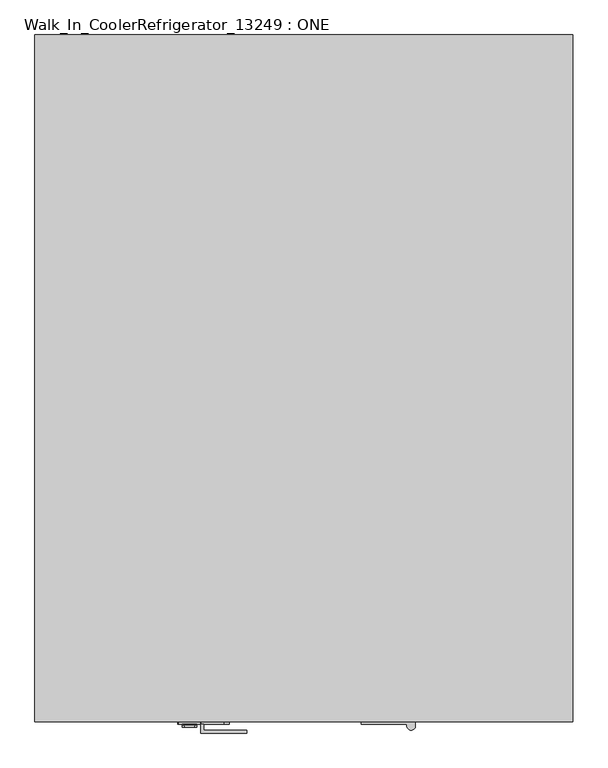
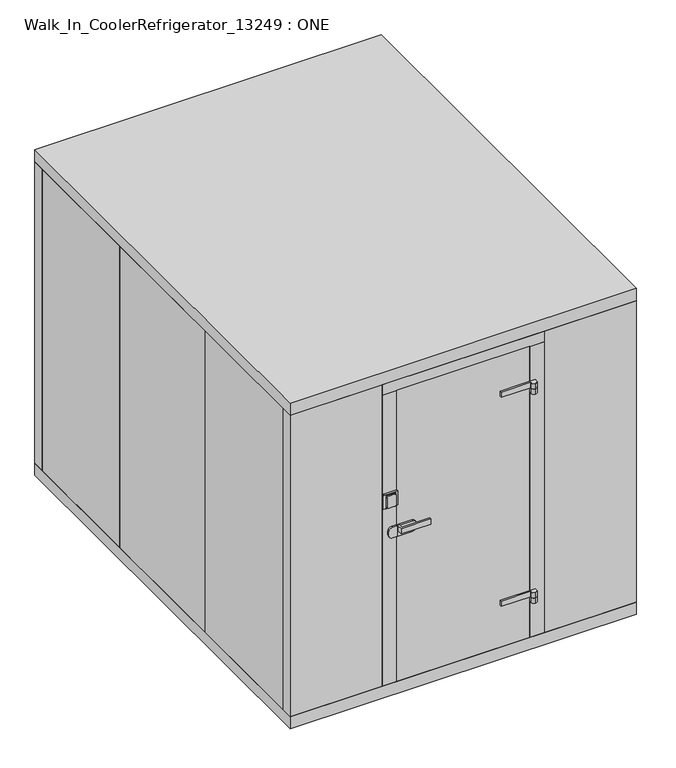
"""IFC4 building model written with IfcOpenShell, lengths in millimetres: proxy geometry, Walk_In_CoolerRefrigerator_13249 : ONE."""

from ifc_helpers import new_model, si_unit, point, frame, frame_2d, origin, origin_with_axes, place, context, project, spatial, polyline, circle_curve, trimmed, segment, composite_curve, outline, extrude, source, transform, mapped, element, save
from ifc_brep_helpers import plane_surface, cylinder_surface, spline_surface, advanced_brep


def walk_in_coolerrefrigerator_13249_one_21fe9a68(model_context):
    return source(origin(), model_context, "Body", "SolidModel", [
        advanced_brep(
        [(-488.8645847, -1549.4, 1390.65), (-527.1354153, -1549.4, 1390.65), (-539.8354153, -1549.4, 1377.95), (-539.8354153, -1549.4, 1314.45), (-527.1354153, -1549.4, 1301.75), (-488.8645847, -1549.4, 1301.75), (-476.1645847, -1549.4, 1314.45), (-476.1645847, -1549.4, 1377.95), (-482.5145847, -1539.875, 1390.65), (-476.1645847, -1539.875, 1384.3), (-476.1645847, -1539.875, 1308.1), (-482.5145847, -1539.875, 1301.75), (-533.4854153, -1539.875, 1301.75), (-539.8354153, -1539.875, 1308.1), (-539.8354153, -1539.875, 1384.3), (-533.4854153, -1539.875, 1390.65)],
        [
            (0, 1),
            (1, 2, circle_curve(frame((-527.1354153, -1549.4, 1377.95), z_axis=(0.0, -1.0, 0.0), x_axis=(-1.0, 0.0, 0.0)), 12.7)),
            (2, 3),
            (3, 4, circle_curve(frame((-527.1354153, -1549.4, 1314.45), z_axis=(0.0, -1.0, 0.0), x_axis=(-1.0, 0.0, 0.0)), 12.7)),
            (4, 5),
            (5, 6, circle_curve(frame((-488.8645847, -1549.4, 1314.45), z_axis=(0.0, -1.0, 0.0), x_axis=(-1.0, 0.0, 0.0)), 12.7)),
            (6, 7),
            (7, 0, circle_curve(frame((-488.8645847, -1549.4, 1377.95), z_axis=(0.0, -1.0, 0.0), x_axis=(-1.0, 0.0, 0.0)), 12.7)),
            (8, 9, circle_curve(frame((-482.5145847, -1539.875, 1384.3), z_axis=(0.0, 1.0, 0.0), x_axis=(-1.0, 0.0, 0.0)), 6.35)),
            (9, 10),
            (10, 11, circle_curve(frame((-482.5145847, -1539.875, 1308.1), z_axis=(0.0, 1.0, 0.0), x_axis=(-1.0, 0.0, 0.0)), 6.35)),
            (11, 12),
            (12, 13, circle_curve(frame((-533.4854153, -1539.875, 1308.1), z_axis=(0.0, 1.0, 0.0), x_axis=(-1.0, 0.0, 0.0)), 6.35)),
            (13, 14),
            (14, 15, circle_curve(frame((-533.4854153, -1539.875, 1384.3), z_axis=(0.0, 1.0, 0.0), x_axis=(-1.0, 0.0, 0.0)), 6.35)),
            (15, 8),
            (15, 1),
            (0, 8),
            (14, 2),
            (13, 3),
            (12, 4),
            (11, 5),
            (10, 6),
            (9, 7),
        ],
        [
            plane_surface(frame((-508.0, -1549.4, 1346.2), z_axis=(0.0, -1.0, 0.0), x_axis=(-1.0, 0.0, 0.0))),
            plane_surface(frame((-508.0, -1539.875, 1346.2), z_axis=(0.0, 1.0, 0.0), x_axis=(-1.0, 0.0, 0.0))),
            plane_surface(frame((-508.0, -1539.875, 1390.65), z_axis=(0.0, 0.0, 1.0), x_axis=(-1.0, 0.0, 0.0))),
            spline_surface(2, 1, [[(-533.4854153, -1539.875, 1390.65), (-527.1354153, -1549.4, 1390.65)], [(-539.8354153000001, -1539.875, 1390.65), (-539.8354153, -1549.4, 1390.65)], [(-539.8354153, -1539.875, 1384.3), (-539.8354153, -1549.4, 1377.95)]], [3, 3], [2, 2], [0.0, 1.0], [0.0, 1.0], weights=[[1.0, 1.0], [0.7071067811865476, 0.7071067811865476], [1.0, 1.0]]),
            plane_surface(frame((-539.8354153, -1539.875, 1346.2), z_axis=(-1.0, 0.0, 0.0), x_axis=(0.0, 0.0, -1.0))),
            spline_surface(2, 1, [[(-539.8354153, -1539.875, 1308.1), (-539.8354153, -1549.4, 1314.45)], [(-539.8354153, -1539.875, 1301.75), (-539.8354153, -1549.4, 1301.75)], [(-533.4854153, -1539.875, 1301.75), (-527.1354153, -1549.4, 1301.75)]], [3, 3], [2, 2], [0.0, 1.0], [0.0, 1.0], weights=[[1.0, 1.0], [0.7071067811865476, 0.7071067811865476], [1.0, 1.0]]),
            plane_surface(frame((-508.0, -1539.875, 1301.75), z_axis=(0.0, 0.0, -1.0), x_axis=(1.0, 0.0, 0.0))),
            spline_surface(2, 1, [[(-482.5145847, -1539.875, 1301.75), (-488.8645847, -1549.4, 1301.75)], [(-476.1645847000001, -1539.875, 1301.75), (-476.1645847, -1549.4, 1301.75)], [(-476.1645847, -1539.875, 1308.1), (-476.1645847, -1549.4, 1314.45)]], [3, 3], [2, 2], [0.0, 1.0], [0.0, 1.0], weights=[[1.0, 1.0], [0.7071067811865476, 0.7071067811865476], [1.0, 1.0]]),
            plane_surface(frame((-476.1645847, -1539.875, 1346.2), z_axis=(1.0, 0.0, 0.0), x_axis=(0.0, 0.0, 1.0))),
            spline_surface(2, 1, [[(-476.1645847, -1539.875, 1384.3), (-476.1645847, -1549.4, 1377.95)], [(-476.1645847, -1539.875, 1390.65), (-476.1645847, -1549.4, 1390.65)], [(-482.5145847, -1539.875, 1390.65), (-488.8645847, -1549.4, 1390.65)]], [3, 3], [2, 2], [0.0, 1.0], [0.0, 1.0], weights=[[1.0, 1.0], [0.7071067811865476, 0.7071067811865476], [1.0, 1.0]]),
        ],
        [
            (0, [[1, 2, 3, 4, 5, 6, 7, 8]]),
            (1, [[9, 10, 11, 12, 13, 14, 15, 16]]),
            (2, [[-16, 17, -1, 18]]),
            (3, [[-15, 19, -2, -17]]),
            (4, [[-14, 20, -3, -19]]),
            (5, [[-13, 21, -4, -20]]),
            (6, [[-12, 22, -5, -21]]),
            (7, [[-11, 23, -6, -22]]),
            (8, [[-10, 24, -7, -23]]),
            (9, [[-9, -18, -8, -24]]),
        ],
    ),
        advanced_brep(
        [(-555.625, -1536.7, 1397.0), (-558.8, -1536.7, 1393.825), (-558.8, -1536.7, 1298.575), (-555.625, -1536.7, 1295.4), (-539.8354153, -1536.7, 1295.4), (-539.8354153, -1536.7, 1397.0), (-460.375, -1536.7, 1295.4), (-457.2, -1536.7, 1298.575), (-457.2, -1536.7, 1393.825), (-460.375, -1536.7, 1397.0), (-476.1645847, -1536.7, 1397.0), (-476.1645847, -1536.7, 1295.4), (-460.375, -1524.0, 1397.0), (-457.2, -1524.0, 1393.825), (-457.2, -1524.0, 1298.575), (-460.375, -1524.0, 1295.4), (-555.625, -1524.0, 1295.4), (-558.8, -1524.0, 1298.575), (-558.8, -1524.0, 1393.825), (-555.625, -1524.0, 1397.0), (-476.1645847, -1539.875, 1390.65), (-539.8354153, -1539.875, 1390.65), (-539.8354153, -1539.875, 1301.75), (-476.1645847, -1539.875, 1301.75)],
        [
            (0, 1, circle_curve(frame((-555.625, -1536.7, 1393.825), z_axis=(0.0, -1.0, 0.0), x_axis=(-1.0, 0.0, 0.0)), 3.175)),
            (1, 2),
            (2, 3, circle_curve(frame((-555.625, -1536.7, 1298.575), z_axis=(0.0, -1.0, 0.0), x_axis=(-1.0, 0.0, 0.0)), 3.175)),
            (3, 4),
            (4, 5),
            (5, 0),
            (6, 7, circle_curve(frame((-460.375, -1536.7, 1298.575), z_axis=(0.0, -1.0, 0.0), x_axis=(-1.0, 0.0, 0.0)), 3.175)),
            (7, 8),
            (8, 9, circle_curve(frame((-460.375, -1536.7, 1393.825), z_axis=(0.0, -1.0, 0.0), x_axis=(-1.0, 0.0, 0.0)), 3.175)),
            (9, 10),
            (10, 11),
            (11, 6),
            (12, 13, circle_curve(frame((-460.375, -1524.0, 1393.825), z_axis=(0.0, 1.0, 0.0), x_axis=(-1.0, 0.0, 0.0)), 3.175)),
            (13, 14),
            (14, 15, circle_curve(frame((-460.375, -1524.0, 1298.575), z_axis=(0.0, 1.0, 0.0), x_axis=(-1.0, 0.0, 0.0)), 3.175)),
            (15, 16),
            (16, 17, circle_curve(frame((-555.625, -1524.0, 1298.575), z_axis=(0.0, 1.0, 0.0), x_axis=(-1.0, 0.0, 0.0)), 3.175)),
            (17, 18),
            (18, 19, circle_curve(frame((-555.625, -1524.0, 1393.825), z_axis=(0.0, 1.0, 0.0), x_axis=(-1.0, 0.0, 0.0)), 3.175)),
            (19, 12),
            (19, 0),
            (5, 10),
            (9, 12),
            (18, 1),
            (17, 2),
            (16, 3),
            (15, 6),
            (11, 4),
            (14, 7),
            (13, 8),
            (20, 21),
            (21, 22),
            (22, 23),
            (23, 20),
            (20, 10),
            (5, 21),
            (4, 22),
            (11, 23),
        ],
        [
            plane_surface(frame((-555.625, -1536.7, 1397.0), z_axis=(0.0, -1.0, 0.0), x_axis=(-1.0, 0.0, 0.0))),
            plane_surface(frame((-555.625, -1524.0, 1397.0), z_axis=(0.0, 1.0, 0.0), x_axis=(1.0, 0.0, 0.0))),
            plane_surface(frame((-460.375, -1536.7, 1397.0), z_axis=(0.0, 0.0, 1.0), x_axis=(0.0, 1.0, 0.0))),
            cylinder_surface(frame((-555.625, -1524.0, 1393.825), z_axis=(0.0, -1.0, 0.0), x_axis=(-1.0, 0.0, 0.0)), 3.175),
            plane_surface(frame((-558.8, -1536.7, 1393.825), z_axis=(-1.0, 0.0, 0.0), x_axis=(0.0, 1.0, 0.0))),
            cylinder_surface(frame((-555.625, -1524.0, 1298.575), z_axis=(0.0, -1.0, 0.0), x_axis=(-1.0, 0.0, 0.0)), 3.175),
            plane_surface(frame((-555.625, -1536.7, 1295.4), z_axis=(0.0, 0.0, -1.0), x_axis=(0.0, 1.0, 0.0))),
            cylinder_surface(frame((-460.375, -1524.0, 1298.575), z_axis=(0.0, -1.0, 0.0), x_axis=(-1.0, 0.0, 0.0)), 3.175),
            plane_surface(frame((-457.2, -1536.7, 1298.575), z_axis=(1.0, 0.0, 0.0), x_axis=(0.0, 1.0, 0.0))),
            cylinder_surface(frame((-460.375, -1524.0, 1393.825), z_axis=(0.0, -1.0, 0.0), x_axis=(-1.0, 0.0, 0.0)), 3.175),
            plane_surface(frame((-508.0, -1539.875, 1346.2), z_axis=(0.0, -1.0, 0.0), x_axis=(-1.0, 0.0, 0.0))),
            plane_surface(frame((-508.0, -1536.7, 1397.0), z_axis=(0.0, -0.8944271909999134, 0.447213595499963), x_axis=(-1.0, 0.0, 0.0))),
            plane_surface(frame((-539.8354153, -1536.7, 1346.2), z_axis=(-1.0, 0.0, 0.0), x_axis=(0.0, 0.0, -1.0))),
            plane_surface(frame((-508.0, -1536.7, 1295.4), z_axis=(0.0, -0.8944271909999666, -0.4472135954998567), x_axis=(1.0, 0.0, 0.0))),
            plane_surface(frame((-476.1645847, -1536.7, 1346.2), z_axis=(1.0, 0.0, 0.0), x_axis=(0.0, 0.0, 1.0))),
        ],
        [
            (0, [[1, 2, 3, 4, 5, 6]]),
            (0, [[7, 8, 9, 10, 11, 12]]),
            (1, [[13, 14, 15, 16, 17, 18, 19, 20]]),
            (2, [[-20, 21, -6, 22, -10, 23]]),
            (3, [[-1, -21, -19, 24]]),
            (4, [[-2, -24, -18, 25]]),
            (5, [[-3, -25, -17, 26]]),
            (6, [[-16, 27, -12, 28, -4, -26]]),
            (7, [[-7, -27, -15, 29]]),
            (8, [[-8, -29, -14, 30]]),
            (9, [[-9, -30, -13, -23]]),
            (10, [[31, 32, 33, 34]]),
            (11, [[-31, 35, -22, 36]]),
            (12, [[-32, -36, -5, 37]]),
            (13, [[-33, -37, -28, 38]]),
            (14, [[-34, -38, -11, -35]]),
        ],
    ),
        extrude(outline(polyline([(-457.2, -1574.8), (-457.2, -1536.7), (-444.5, -1536.7), (-444.5, -1562.1), (-254.0, -1562.1), (-254.0, -1574.8), (-457.2, -1574.8)])), frame((0.0, 0.0, 1104.9), z_axis=(0.0, 0.0, 1.0), x_axis=(1.0, 0.0, 0.0)), (0.0, 0.0, 1.0), 38.1),
        extrude(outline(composite_curve([segment(polyline([(1066.8, -457.2), (1066.8, -355.6)]), True, "CONTINUOUS"), segment(trimmed(circle_curve(frame_2d((1092.2, -355.6)), 25.4), [point((1066.8, -355.6))], [point((1092.2, -330.2))], False, "CARTESIAN"), True, "CONTINUOUS"), segment(polyline([(1092.2, -330.2), (1117.6, -330.2)]), True, "CONTINUOUS"), segment(trimmed(circle_curve(frame_2d((1117.6, -355.6)), 25.4), [point((1117.6, -330.2))], [point((1143.0, -355.6))], False, "CARTESIAN"), True, "CONTINUOUS"), segment(polyline([(1143.0, -355.6), (1143.0, -457.2), (1066.8, -457.2)]), True, "CONTINUOUS")], self_intersect=False)), frame((0.0, -1536.7, 0.0), z_axis=(0.0, 1.0, 0.0), x_axis=(0.0, 0.0, 1.0)), (0.0, 0.0, 1.0), 12.7),
        extrude(outline(composite_curve([segment(polyline([(1066.8, -457.2), (1143.0, -457.2), (1143.0, -495.3)]), True, "CONTINUOUS"), segment(trimmed(circle_curve(frame_2d((1117.6, -495.3)), 25.4), [point((1143.0, -495.3))], [point((1117.6, -520.7))], False, "CARTESIAN"), True, "CONTINUOUS"), segment(polyline([(1117.6, -520.7), (1092.2, -520.7)]), True, "CONTINUOUS"), segment(trimmed(circle_curve(frame_2d((1092.2, -495.3)), 25.4), [point((1092.2, -520.7))], [point((1066.8, -495.3))], False, "CARTESIAN"), True, "CONTINUOUS"), segment(polyline([(1066.8, -495.3), (1066.8, -457.2)]), True, "CONTINUOUS")], self_intersect=False)), frame((0.0, -1536.7, 0.0), z_axis=(0.0, 1.0, 0.0), x_axis=(0.0, 0.0, 1.0)), (0.0, 0.0, 1.0), 12.7),
        extrude(outline(composite_curve([segment(polyline([(254.0, -1536.7), (254.0, -1524.0), (495.3, -1524.0), (495.3, -1543.05)]), True, "CONTINUOUS"), segment(trimmed(circle_curve(frame_2d((476.25, -1543.05)), 19.05), [point((495.3, -1543.05))], [point((476.25, -1562.1))], False, "CARTESIAN"), True, "CONTINUOUS"), segment(trimmed(circle_curve(frame_2d((476.25, -1543.05)), 19.05), [point((476.25, -1562.1))], [point((457.2, -1543.05))], False, "CARTESIAN"), True, "CONTINUOUS"), segment(polyline([(457.2, -1543.05), (457.2, -1536.7), (254.0, -1536.7)]), True, "CONTINUOUS")], self_intersect=False)), frame((0.0, 0.0, 304.8), z_axis=(0.0, 0.0, 1.0), x_axis=(1.0, 0.0, 0.0)), (0.0, 0.0, 1.0), 38.1),
        extrude(outline(composite_curve([segment(polyline([(457.2, -1543.05), (457.2, -1524.0), (495.3, -1524.0), (495.3, -1543.05)]), True, "CONTINUOUS"), segment(trimmed(circle_curve(frame_2d((476.25, -1543.05)), 19.05), [point((495.3, -1543.05))], [point((476.25, -1562.1))], False, "CARTESIAN"), True, "CONTINUOUS"), segment(trimmed(circle_curve(frame_2d((476.25, -1543.05)), 19.05), [point((476.25, -1562.1))], [point((457.2, -1543.05))], False, "CARTESIAN"), True, "CONTINUOUS")], self_intersect=False)), frame((0.0, 0.0, 266.7), z_axis=(0.0, 0.0, 1.0), x_axis=(1.0, 0.0, 0.0)), (0.0, 0.0, 1.0), 38.1),
        extrude(outline(composite_curve([segment(polyline([(495.3, -1524.0), (495.3, -1543.05)]), True, "CONTINUOUS"), segment(trimmed(circle_curve(frame_2d((476.25, -1543.05)), 19.05), [point((495.3, -1543.05))], [point((476.25, -1562.1))], False, "CARTESIAN"), True, "CONTINUOUS"), segment(trimmed(circle_curve(frame_2d((476.25, -1543.05)), 19.05), [point((476.25, -1562.1))], [point((457.2, -1543.05))], False, "CARTESIAN"), True, "CONTINUOUS"), segment(polyline([(457.2, -1543.05), (457.2, -1536.7), (254.0, -1536.7), (254.0, -1524.0), (495.3, -1524.0)]), True, "CONTINUOUS")], self_intersect=False)), frame((0.0, 0.0, 1828.8), z_axis=(0.0, 0.0, 1.0), x_axis=(1.0, 0.0, 0.0)), (0.0, 0.0, 1.0), 38.1),
        extrude(outline(composite_curve([segment(polyline([(457.2, -1543.05), (457.2, -1524.0), (495.3, -1524.0), (495.3, -1543.05)]), True, "CONTINUOUS"), segment(trimmed(circle_curve(frame_2d((476.25, -1543.05)), 19.05), [point((495.3, -1543.05))], [point((476.25, -1562.1))], False, "CARTESIAN"), True, "CONTINUOUS"), segment(trimmed(circle_curve(frame_2d((476.25, -1543.05)), 19.05), [point((476.25, -1562.1))], [point((457.2, -1543.05))], False, "CARTESIAN"), True, "CONTINUOUS")], self_intersect=False)), frame((0.0, 0.0, 1790.7), z_axis=(0.0, 0.0, 1.0), x_axis=(1.0, 0.0, 0.0)), (0.0, 0.0, 1.0), 38.1),
        extrude(outline(polyline([(457.2, -1435.1), (457.2, -1524.0), (-457.2, -1524.0), (-457.2, -1435.1), (457.2, -1435.1)])), origin_with_axes(), (0.0, 0.0, 1.0), 2120.9),
        extrude(outline(polyline([(558.8, -1435.1), (558.8, -1524.0), (-558.8, -1524.0), (-558.8, -1435.1), (558.8, -1435.1)])), frame((0.0, 0.0, 2120.9), z_axis=(0.0, 0.0, 1.0), x_axis=(1.0, 0.0, 0.0)), (0.0, 0.0, 1.0), 76.2),
        extrude(outline(polyline([(-558.8, -1435.1), (-457.2, -1435.1), (-457.2, -1524.0), (-558.8, -1524.0), (-558.8, -1435.1)])), origin_with_axes(), (0.0, 0.0, 1.0), 2120.9),
        extrude(outline(polyline([(558.8, -1435.1), (558.8, -1524.0), (457.2, -1524.0), (457.2, -1435.1), (558.8, -1435.1)])), origin_with_axes(), (0.0, 0.0, 1.0), 2120.9),
        extrude(outline(polyline([(1193.8, -1524.0), (-1193.8, -1524.0), (-1193.8, 1524.0), (1193.8, 1524.0), (1193.8, -1524.0)])), frame((0.0, 0.0, 2197.1), z_axis=(0.0, 0.0, 1.0), x_axis=(1.0, 0.0, 0.0)), (0.0, 0.0, 1.0), 88.9),
        extrude(outline(polyline([(-1193.8, -508.0), (-1104.9, -508.0), (-1104.9, -1435.1), (-1193.8, -1435.1), (-1193.8, -508.0)])), origin_with_axes(), (0.0, 0.0, 1.0), 2197.1),
        extrude(outline(polyline([(1104.9, -508.0), (1193.8, -508.0), (1193.8, -1435.1), (1104.9, -1435.1), (1104.9, -508.0)])), origin_with_axes(), (0.0, 0.0, 1.0), 2197.1),
        extrude(outline(polyline([(1104.9, 508.0), (1193.8, 508.0), (1193.8, -508.0), (1104.9, -508.0), (1104.9, 508.0)])), origin_with_axes(), (0.0, 0.0, 1.0), 2197.1),
        extrude(outline(polyline([(-1193.8, 508.0), (-1104.9, 508.0), (-1104.9, -508.0), (-1193.8, -508.0), (-1193.8, 508.0)])), origin_with_axes(), (0.0, 0.0, 1.0), 2197.1),
        extrude(outline(polyline([(-1193.8, 1435.1), (-1104.9, 1435.1), (-1104.9, 508.0), (-1193.8, 508.0), (-1193.8, 1435.1)])), origin_with_axes(), (0.0, 0.0, 1.0), 2197.1),
        extrude(outline(polyline([(1104.9, 1435.1), (1193.8, 1435.1), (1193.8, 508.0), (1104.9, 508.0), (1104.9, 1435.1)])), origin_with_axes(), (0.0, 0.0, 1.0), 2197.1),
        extrude(outline(polyline([(-457.2, 1435.1), (-457.2, 1524.0), (457.2, 1524.0), (457.2, 1435.1), (-457.2, 1435.1)])), origin_with_axes(), (0.0, 0.0, 1.0), 2197.1),
        extrude(outline(polyline([(457.2, 1435.1), (457.2, 1524.0), (1193.8, 1524.0), (1193.8, 1435.1), (457.2, 1435.1)])), origin_with_axes(), (0.0, 0.0, 1.0), 2197.1),
        extrude(outline(polyline([(-457.2, 1435.1), (-1193.8, 1435.1), (-1193.8, 1524.0), (-457.2, 1524.0), (-457.2, 1435.1)])), origin_with_axes(), (0.0, 0.0, 1.0), 2197.1),
        extrude(outline(polyline([(558.8, -1435.1), (1193.8, -1435.1), (1193.8, -1524.0), (558.8, -1524.0), (558.8, -1435.1)])), origin_with_axes(), (0.0, 0.0, 1.0), 2197.1),
        extrude(outline(polyline([(-558.8, -1435.1), (-558.8, -1524.0), (-1193.8, -1524.0), (-1193.8, -1435.1), (-558.8, -1435.1)])), origin_with_axes(), (0.0, 0.0, 1.0), 2197.1),
        extrude(outline(polyline([(1193.8, 1524.0), (1193.8, -1524.0), (-1193.8, -1524.0), (-1193.8, 1524.0), (1193.8, 1524.0)])), frame((0.0, 0.0, -88.9), z_axis=(0.0, 0.0, 1.0), x_axis=(1.0, 0.0, 0.0)), (0.0, 0.0, 1.0), 88.9),
    ])


if __name__ == "__main__":
    model = new_model("IFC4")
    model_context = context("Model", 3, world=origin())
    ifc_project = project(units=[si_unit("LENGTHUNIT", "METRE", prefix="MILLI")], contexts=[model_context])
    site = spatial("IfcSite", under=ifc_project)
    building = spatial("IfcBuilding", under=site)
    placement = place(None, origin())
    walk_in_coolerrefrigerator_13249_one_shape = walk_in_coolerrefrigerator_13249_one_21fe9a68(model_context)
    element("IfcBuildingElementProxy", 1, Name="Walk_In_CoolerRefrigerator_13249 : ONE", ObjectType="Walk_In_CoolerRefrigerator_13249 : ONE", at=placement, inside=building, context=model_context, shape_type="MappedRepresentation", body=[
        mapped(walk_in_coolerrefrigerator_13249_one_shape, transform((0.0, 0.0, 0.0), x_axis=(1.0, 0.0, 0.0), y_axis=(0.0, 1.0, 0.0), z_axis=(0.0, 0.0, 1.0))),
    ])
    save(model, "model.ifc")

# Revit data of these elements
# Type "Walk_In_CoolerRefrigerator_13249 : ONE"
#   Width = 7' - 10"
#   Height = 7' - 6"
#   Door Width = 3' - 0"
#   Door Height = 6' - 11 1/2"
#   Depth = 10' - 0"
#   DSPW = 2' - 1"
#   Refrigerator Panel [instance default] = WALK-IN COOLER
# Element 1 (IfcBuildingElementProxy, "Walk_In_CoolerRefrigerator_13249 : ONE")
#   Materials on its faces: "WALK-IN COOLER", "FireAlarmDevice_Casement", "FireAlarmDevice_ClearPlastic"
# Materials
#   "WALK-IN COOLER": class "Metal", colour RGB 233 233 233, transparency 0, Cost = 0
#   "FireAlarmDevice_Casement": class "Paint", colour RGB 242 242 255, transparency 0
#   "FireAlarmDevice_ClearPlastic": class "Plastic", colour RGB 255 255 255, transparency 0.75
